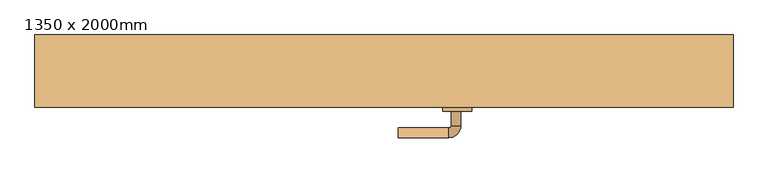
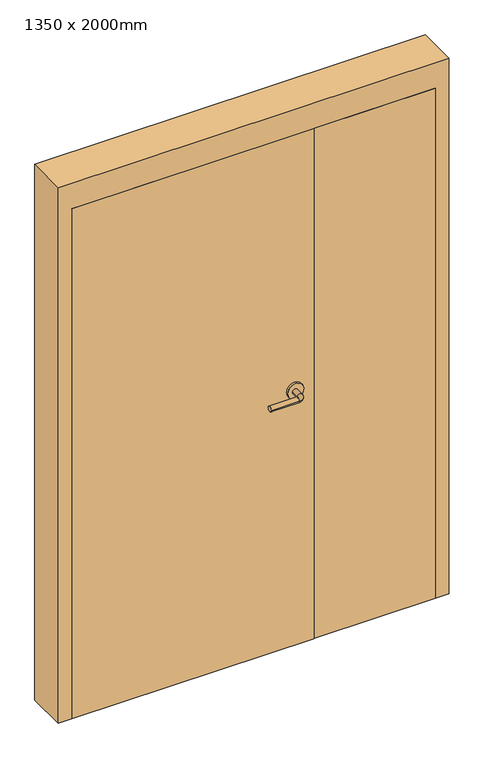
"""IFC4 building model written with IfcOpenShell, lengths in millimetres: door geometry, Porta-Passagem-Irregular-Nivelada : 1350 x 2000mm."""

from ifc_helpers import new_model, si_unit, point, frame, frame_2d, origin, origin_with_axes, place, context, project, spatial, polyline, circle_curve, ellipse_curve, trimmed, segment, composite_curve, outline, extrude, faceted_brep, source, transform, mapped, element, save
from ifc_brep_helpers import plane_surface, cylinder_surface, revolved_surface, advanced_brep


def door_1350_x_2000mm_5ea6081c(model_context):
    return source(origin(), model_context, "Body", "SolidModel", [
        advanced_brep(
        [(159.59375, -28.35, 1000.0), (139.59375, -28.35, 1000.0), (139.59375, 1.65, 1000.0), (159.59375, 1.65, 1000.0), (134.59375, 6.65, 1000.0), (134.59375, 26.65, 1000.0), (29.59375, 26.65, 1000.0), (29.59375, 6.65, 1000.0)],
        [
            (0, 1, circle_curve(frame((149.59375, -28.35, 1000.0), z_axis=(0.0, -1.0, 0.0), x_axis=(-1.0, 0.0, 0.0)), 10.0)),
            (1, 0, circle_curve(frame((149.59375, -28.35, 1000.0), z_axis=(0.0, -1.0, 0.0), x_axis=(-1.0, 0.0, 0.0)), 10.0)),
            (1, 2),
            (2, 3, circle_curve(frame((149.59375, 1.65, 1000.0), z_axis=(0.0, -1.0, 0.0), x_axis=(-1.0, 0.0, 0.0)), 10.0)),
            (3, 0),
            (3, 2, circle_curve(frame((149.59375, 1.65, 1000.0), z_axis=(0.0, -1.0, 0.0), x_axis=(-1.0, 0.0, 0.0)), 10.0)),
            (4, 5, circle_curve(frame((134.59375, 16.65, 1000.0), z_axis=(1.0, 0.0, 0.0), x_axis=(0.0, -1.0, 0.0)), 10.0)),
            (5, 3, circle_curve(frame((134.59375, 1.65, 1000.0), z_axis=(0.0, 0.0, -1.0), x_axis=(1.0, 0.0, 0.0)), 25.0)),
            (2, 4, circle_curve(frame((134.59375, 1.65, 1000.0), z_axis=(0.0, 0.0, 1.0), x_axis=(1.0, 0.0, 0.0)), 5.0)),
            (5, 4, circle_curve(frame((134.59375, 16.65, 1000.0), z_axis=(1.0, 0.0, 0.0), x_axis=(0.0, -1.0, 0.0)), 10.0)),
            (6, 7, circle_curve(frame((29.59375, 16.65, 1000.0), z_axis=(-1.0, 0.0, 0.0), x_axis=(0.0, -1.0, 0.0)), 10.0)),
            (7, 6, circle_curve(frame((29.59375, 16.65, 1000.0), z_axis=(-1.0, 0.0, 0.0), x_axis=(0.0, -1.0, 0.0)), 10.0)),
            (4, 7),
            (6, 5),
        ],
        [
            plane_surface(frame((149.59375, -28.35, 1000.0), z_axis=(0.0, -1.0, 0.0), x_axis=(0.0, 0.0, 1.0))),
            cylinder_surface(frame((149.59375, -28.35, 1000.0), z_axis=(0.0, -1.0, 0.0), x_axis=(-1.0, 0.0, 0.0)), 10.0),
            revolved_surface(trimmed(ellipse_curve(frame((149.59375, 1.65, 1000.0), z_axis=(0.0, 1.0, 0.0), x_axis=(-1.0, 0.0, 0.0)), 10.0, 10.0), [point((159.59375, 1.65, 1000.0))], [point((139.59375, 1.65, 1000.0))], True, "CARTESIAN"), (134.59375, 1.65, 1000.0), (0.0, 0.0, -1.0)),
            revolved_surface(trimmed(ellipse_curve(frame((149.59375, 1.65, 1000.0), z_axis=(0.0, 1.0, 0.0), x_axis=(-1.0, 0.0, 0.0)), 10.0, 10.0), [point((139.59375, 1.65, 1000.0))], [point((159.59375, 1.65, 1000.0))], True, "CARTESIAN"), (134.59375, 1.65, 1000.0), (0.0, 0.0, -1.0)),
            plane_surface(frame((29.59375, 16.65, 1000.0), z_axis=(-1.0, 0.0, 0.0), x_axis=(0.0, 0.0, 1.0))),
            cylinder_surface(frame((134.59375, 16.65, 1000.0), z_axis=(1.0, 0.0, 0.0), x_axis=(0.0, -1.0, 0.0)), 10.0),
        ],
        [
            (0, [[1, 2]]),
            (1, [[3, 4, 5, -2]]),
            (1, [[-5, 6, -3, -1]]),
            (2, [[7, 8, -4, 9]]),
            (3, [[10, -9, -6, -8]]),
            (4, [[11, 12]]),
            (5, [[13, -11, 14, -7]]),
            (5, [[-14, -12, -13, -10]]),
        ],
    ),
        extrude(outline(composite_curve([segment(trimmed(circle_curve(frame_2d((1000.0, 152.09375)), 30.0), [point((1000.0, 182.09375))], [point((1000.0, 122.09375))], False, "CARTESIAN"), True, "CONTINUOUS"), segment(trimmed(circle_curve(frame_2d((1000.0, 152.09375)), 30.0), [point((1000.0, 122.09375))], [point((1000.0, 182.09375))], False, "CARTESIAN"), True, "CONTINUOUS")], self_intersect=False)), frame((0.0, -36.35, 0.0), z_axis=(0.0, 1.0, 0.0), x_axis=(0.0, 0.0, 1.0)), (0.0, 0.0, 1.0), 8.0),
        advanced_brep(
        [(159.59375, -89.35, 1000.0), (139.59375, -89.35, 1000.0), (159.59375, -119.35, 1000.0), (139.59375, -119.35, 1000.0), (134.59375, -124.35, 1000.0), (134.59375, -144.35, 1000.0), (29.59375, -144.35, 1000.0), (29.59375, -124.35, 1000.0)],
        [
            (0, 1, circle_curve(frame((149.59375, -89.35, 1000.0), z_axis=(0.0, 1.0, 0.0), x_axis=(-1.0, 0.0, 0.0)), 10.0)),
            (1, 0, circle_curve(frame((149.59375, -89.35, 1000.0), z_axis=(0.0, 1.0, 0.0), x_axis=(-1.0, 0.0, 0.0)), 10.0)),
            (0, 2),
            (2, 3, circle_curve(frame((149.59375, -119.35, 1000.0), z_axis=(0.0, 1.0, 0.0), x_axis=(-1.0, 0.0, 0.0)), 10.0)),
            (3, 1),
            (3, 2, circle_curve(frame((149.59375, -119.35, 1000.0), z_axis=(0.0, 1.0, 0.0), x_axis=(-1.0, 0.0, 0.0)), 10.0)),
            (4, 3, circle_curve(frame((134.59375, -119.35, 1000.0), z_axis=(0.0, 0.0, 1.0), x_axis=(1.0, 0.0, 0.0)), 5.0)),
            (2, 5, circle_curve(frame((134.59375, -119.35, 1000.0), z_axis=(0.0, 0.0, -1.0), x_axis=(1.0, 0.0, 0.0)), 25.0)),
            (5, 4, circle_curve(frame((134.59375, -134.35, 1000.0), z_axis=(1.0, 0.0, 0.0), x_axis=(0.0, 1.0, 0.0)), 10.0)),
            (4, 5, circle_curve(frame((134.59375, -134.35, 1000.0), z_axis=(1.0, 0.0, 0.0), x_axis=(0.0, 1.0, 0.0)), 10.0)),
            (6, 7, circle_curve(frame((29.59375, -134.35, 1000.0), z_axis=(-1.0, 0.0, 0.0), x_axis=(0.0, 1.0, 0.0)), 10.0)),
            (7, 6, circle_curve(frame((29.59375, -134.35, 1000.0), z_axis=(-1.0, 0.0, 0.0), x_axis=(0.0, 1.0, 0.0)), 10.0)),
            (5, 6),
            (7, 4),
        ],
        [
            plane_surface(frame((149.59375, -89.35, 1000.0), z_axis=(0.0, 1.0, 0.0), x_axis=(0.0, 0.0, 1.0))),
            cylinder_surface(frame((149.59375, -89.35, 1000.0), z_axis=(0.0, 1.0, 0.0), x_axis=(-1.0, 0.0, 0.0)), 10.0),
            revolved_surface(trimmed(ellipse_curve(frame((149.59375, -119.35, 1000.0), z_axis=(0.0, 1.0, 0.0), x_axis=(-1.0, 0.0, 0.0)), 10.0, 10.0), [point((159.59375, -119.35, 1000.0))], [point((139.59375, -119.35, 1000.0))], True, "CARTESIAN"), (134.59375, -119.35, 1000.0), (0.0, 0.0, -1.0)),
            revolved_surface(trimmed(ellipse_curve(frame((149.59375, -119.35, 1000.0), z_axis=(0.0, 1.0, 0.0), x_axis=(-1.0, 0.0, 0.0)), 10.0, 10.0), [point((139.59375, -119.35, 1000.0))], [point((159.59375, -119.35, 1000.0))], True, "CARTESIAN"), (134.59375, -119.35, 1000.0), (0.0, 0.0, -1.0)),
            plane_surface(frame((29.59375, -134.35, 1000.0), z_axis=(-1.0, 0.0, 0.0), x_axis=(0.0, 0.0, 1.0))),
            cylinder_surface(frame((134.59375, -134.35, 1000.0), z_axis=(1.0, 0.0, 0.0), x_axis=(0.0, 1.0, 0.0)), 10.0),
        ],
        [
            (0, [[1, 2]]),
            (1, [[-1, 3, 4, 5]]),
            (1, [[-2, -5, 6, -3]]),
            (2, [[7, -4, 8, 9]]),
            (3, [[-8, -6, -7, 10]]),
            (4, [[11, 12]]),
            (5, [[-9, 13, -12, 14]]),
            (5, [[-10, -14, -11, -13]]),
        ],
    ),
        extrude(outline(composite_curve([segment(trimmed(circle_curve(frame_2d((1000.0, 152.09375)), 30.0), [point((1000.0, 182.09375))], [point((1000.0, 122.09375))], False, "CARTESIAN"), True, "CONTINUOUS"), segment(trimmed(circle_curve(frame_2d((1000.0, 152.09375)), 30.0), [point((1000.0, 122.09375))], [point((1000.0, 182.09375))], False, "CARTESIAN"), True, "CONTINUOUS")], self_intersect=False)), frame((0.0, -89.35, 0.0), z_axis=(0.0, 1.0, 0.0), x_axis=(0.0, 0.0, 1.0)), (0.0, 0.0, 1.0), 8.0),
        extrude(outline(polyline([(675.0, -36.35), (675.0, -81.35), (226.6, -81.35), (226.6, -36.35), (675.0, -36.35)])), origin_with_axes(), (0.0, 0.0, 1.0), 2000.0),
        faceted_brep([(675.0, -31.5875, 0.0), (659.125, -31.5875, 0.0), (659.125, 19.4375, 0.0), (675.0, 19.4375, 0.0), (675.0, 68.65, 0.0), (725.0, 68.65, 0.0), (725.0, -81.35, 0.0), (675.0, -81.35, 0.0), (675.0, -81.35, 2000.0), (675.0, -31.5875, 2000.0), (725.0, -81.35, 2100.0), (-725.0, -81.35, 2100.0), (-725.0, -81.35, 0.0), (-675.0, -81.35, 0.0), (-675.0, -81.35, 2000.0), (725.0, 68.65, 2100.0), (675.0, 68.65, 2000.0), (-675.0, 68.65, 2000.0), (-675.0, 68.65, 0.0), (-725.0, 68.65, 0.0), (-725.0, 68.65, 2100.0), (675.0, 19.4375, 2000.0), (659.125, 19.4375, 1984.125), (-659.125, 19.4375, 1984.125), (-659.125, 19.4375, 0.0), (-675.0, 19.4375, 0.0), (-675.0, 19.4375, 2000.0), (659.125, -31.5875, 1984.125), (-675.0, -31.5875, 2000.0), (-675.0, -31.5875, 0.0), (-659.125, -31.5875, 0.0), (-659.125, -31.5875, 1984.125)], [[[0, 1, 2, 3, 4, 5, 6, 7]], [[7, 8, 9, 0]], [[6, 10, 11, 12, 13, 14, 8, 7]], [[5, 15, 10, 6]], [[4, 16, 17, 18, 19, 20, 15, 5]], [[3, 21, 16, 4]], [[2, 22, 23, 24, 25, 26, 21, 3]], [[1, 27, 22, 2]], [[0, 9, 28, 29, 30, 31, 27, 1]], [[8, 14, 28, 9]], [[16, 21, 26, 17]], [[22, 27, 31, 23]], [[12, 19, 18, 25, 24, 30, 29, 13]], [[13, 29, 28, 14]], [[11, 20, 19, 12]], [[17, 26, 25, 18]], [[23, 31, 30, 24]], [[15, 20, 11, 10]]]),
        extrude(outline(polyline([(223.4, -36.35), (223.4, -81.35), (-675.0, -81.35), (-675.0, -36.35), (223.4, -36.35)])), origin_with_axes(), (0.0, 0.0, 1.0), 2000.0),
    ])


if __name__ == "__main__":
    model = new_model("IFC4")
    model_context = context("Model", 3, world=origin())
    ifc_project = project(units=[si_unit("LENGTHUNIT", "METRE", prefix="MILLI")], contexts=[model_context])
    site = spatial("IfcSite", under=ifc_project)
    building = spatial("IfcBuilding", under=site)
    placement = place(None, origin())
    door_1350_x_2000mm_shape = door_1350_x_2000mm_5ea6081c(model_context)
    element("IfcDoor", 1, ObjectType="Porta-Passagem-Irregular-Nivelada : 1350 x 2000mm", at=placement, inside=building, context=model_context, shape_type="MappedRepresentation", body=[
        mapped(door_1350_x_2000mm_shape, transform((0.0, 0.0, 0.0), x_axis=(1.0, 0.0, 0.0), y_axis=(0.0, 1.0, 0.0), z_axis=(0.0, 0.0, 1.0))),
    ])
    save(model, "model.ifc")

# Revit data of these elements
# Project information
#   MCI_ProjInf_tipo_de_projeto = "Residêncial"
#   Data de emissão do projeto = "Data de emissão"
#   Status do projeto = "Status do projeto"
#   Nome do cliente = "Proprietário"
#   Endereço do projeto = "Insira aqui o endereço"
#   Nome do projeto = "Nome do projeto"
#   Número do projeto = "0001"
# Type "Porta-Passagem-Irregular-Nivelada : 1350 x 2000mm"
#   Type Mark = "48"
#   Assembly Code = "C1020300"
#   Analytic Construction = "Madeira"
#   Painel com largura larga = 0.900 m
#   W = 0.450 m
#   Thickness = 0.045 m
#   Thermal Resistance (R) = 0.455703 (m²·K)/W
#   Ângulo de abertura [instance default] = 90.00°
#   Altura do traçado = 1.000 m
#   Rough Width [instance default] = 1.450 m
#   Rough Height [instance default] = 2.100 m
#   Altura da abertura da moldura de alvenaria [instance default] = 0.100 m
#   Largura da abertura da moldura de alvenaria [instance default] = 0.100 m
#   Cálculo da inserção [instance default] = 0.105 m
#   Inserção de alvenaria [instance default] = 0.025 m
#   Height = 2.000 m
#   Width = 1.350 m
#   Heat Transfer Coefficient (U) = 2.19465 W/(m²·K)
#   Profundidade da moldura de alvenaria = 0.150 m
#   MCT_Portas_tetra_chave [instance default] = yes
#   Define Thermal Properties by = 1
#   Moldura de alvenaria [instance default] = yes
#   Moldura de Dry Wall [instance default] = no
#   Material do painel = Madeira - Bétula
#   Material da moldura = Metal - Acabamento de pintura - Cinza
#   Material da maçaneta = Alumín. 1
#   Visual Light Transmittance = 0
#   Solar Heat Gain Coefficient = 0
#   Wall Closure = (empty or 0)
#   Function = (empty or 0)
# Element 1 (IfcDoor, "Porta-Passagem-Irregular-Nivelada : 1350 x 2000mm")
#   Materials on its faces: "Alumín. 1", "Metal - Acabamento de pintura - Cinza", "Madeira - Bétula"
# Materials
#   "Madeira - Bétula": class "Madeira", colour RGB 166 116 52, transparency 0, Cost = 0
#   "Metal - Acabamento de pintura - Cinza": class "Pintura", colour RGB 104 104 104, transparency 0, Cost = 0
#   "Alumín. 1": class "Metal", colour RGB 244 244 244, transparency 0, Description = "Alumín. 6061", Cost = 0
